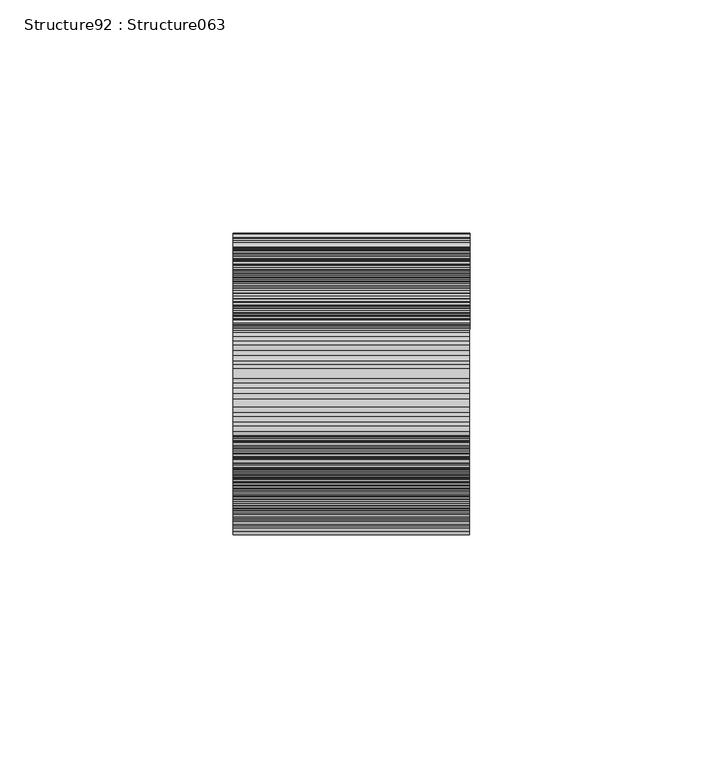
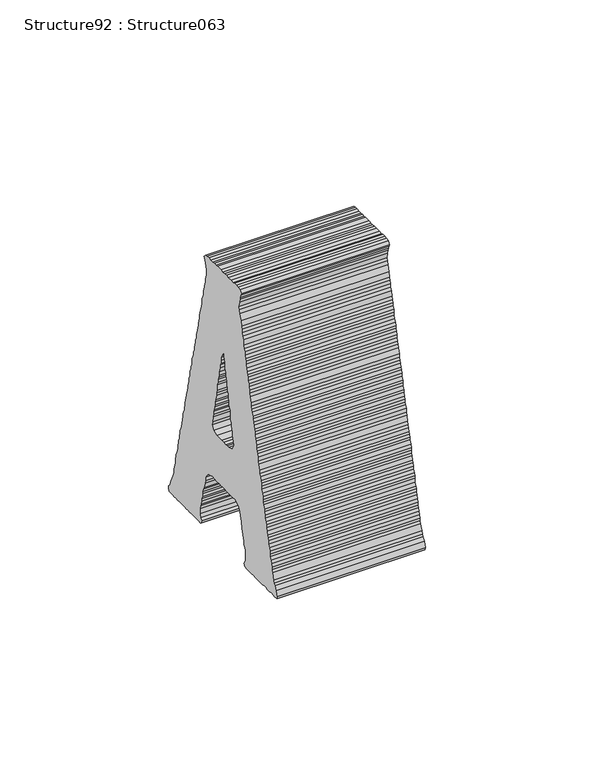
"""IFC4 building model written with IfcOpenShell, lengths in millimetres: proxy geometry, Structure92 : Structure063."""

from ifc_helpers import new_model, si_unit, frame, origin, place, context, project, spatial, polyline, outline, extrude, source, transform, mapped, element, save


def structure92_structure063_1dc17f56(model_context):
    return source(origin(), model_context, "Body", "SweptSolid", [
        extrude(outline(polyline([(0.9094651, 0.0), (2.0811665, -0.5187795), (2.9906316, -0.6522104), (4.1562841, -0.7806598), (5.1991801, -1.1663641), (5.9748585, -1.299795), (7.1504738, -1.690125), (8.1894559, -1.690125), (9.3551083, -2.0804548), (10.2645735, -2.3373539), (11.4362748, -2.5992343), (12.3453841, -2.856489), (13.3818755, -2.9849385), (14.1582655, -3.3752685), (15.4626861, -3.5086994), (16.3721513, -3.5086994), (17.5385154, -3.7705798), (19.491944, -4.4131831), (20.2718921, -4.6750635), (21.3101626, -4.9369439), (22.3470097, -4.9369439), (23.2561191, -5.1988243), (24.4278204, -5.5891542), (25.4700048, -5.9745026), (26.6363689, -5.9745026), (27.4124031, -6.3651884), (28.7175354, -6.6270688), (30.535754, -7.0173988), (31.5743802, -7.1458482), (32.7400327, -7.4077286), (33.6555467, -7.7934329), (35.4741211, -7.7934329), (36.5102567, -7.5361781), (37.5492387, -7.2742977), (38.3288311, -6.8839678), (39.3671015, -6.3651884), (40.4099976, -7.2742977), (40.5395145, -8.1837628), (40.5395145, -9.0978536), (40.2826155, -10.2642177), (40.2826155, -11.3021323), (40.5395145, -12.4731221), (40.4099976, -13.2491562), (40.5395145, -14.1632469), (40.5395145, -16.2390762), (40.2826155, -17.2816164), (40.2826155, -18.319531), (40.5395145, -19.4858951), (40.4099976, -20.6618662), (40.4099976, -22.3470097), (40.2826155, -23.5183552), (40.5395145, -24.422839), (40.5395145, -25.5988102), (40.4099976, -26.5032939), (40.2826155, -27.6696579), (39.2382962, -28.4552992), (38.3288311, -27.9315383), (37.4197218, -27.6696579), (36.6397736, -27.5458341), (35.4741211, -27.2839537), (33.5199809, -26.8936237), (32.6112274, -27.1555041), (31.4448633, -27.4173846), (29.3636968, -28.1934188), (27.545834, -28.4552992), (26.5089869, -28.7121982), (25.3372855, -28.8456291), (24.2943895, -29.1025281), (23.2561191, -29.6216633), (21.3101626, -29.7501128), (20.2718921, -30.0119931), (19.491944, -30.535754), (18.3202426, -30.535754), (17.2816164, -30.9214583), (16.3721513, -31.1783573), (15.3356599, -31.1783573), (14.1582655, -31.4402377), (13.1253323, -31.8305676), (12.2158672, -32.2208975), (11.4362748, -32.3543284), (10.2645735, -32.4827779), (9.3551083, -32.8684823), (8.1894559, -32.8684823), (7.1504738, -33.2588121), (6.2374505, -33.392243), (5.0714422, -33.649142), (3.2475306, -34.2967267), (2.0811665, -34.2967267), (1.1720572, -34.5586071), (0.1334309, -34.8204876), (-1.0382704, -35.3392669), (-1.8178628, -35.4726979), (-2.8568449, -35.7295969), (-3.8990293, -35.8630278), (-5.0653934, -36.2487321), (-5.8471206, -36.5106126), (-7.0166871, -36.5106126), (-8.1826954, -36.9009424), (-8.9644226, -37.0293919), (-10.1364798, -37.4197219), (-11.1690572, -37.5485272), (-12.2115974, -37.6769766), (-12.9915456, -37.938857), (-14.03373, -38.3291869), (-15.3292552, -38.4576365), (-16.3678815, -38.7195168), (-18.1861001, -39.1098467), (-19.3581573, -39.3671016), (-20.2672666, -39.7574315), (-21.4371888, -40.0143304), (-22.2189161, -40.2762109), (-23.1223323, -40.5380913), (-24.1648726, -40.5380913), (-25.465735, -41.052245), (-26.5025822, -41.3141255), (-27.4173846, -41.4475564), (-28.4560108, -41.4475564), (-29.235959, -41.7044554), (-30.5311284, -42.0947853), (-31.3110766, -42.2282162), (-32.3536168, -42.6139205), (-33.5214042, -42.6139205), (-34.4308693, -43.1326999), (-35.3399786, -43.3945803), (-36.37647, -43.3945803), (-37.5424783, -43.6564607), (-38.7202285, -44.0467907), (-39.6236447, -44.3040454), (-40.405372, -44.5609444), (-41.5752942, -44.6943753), (-42.6139205, -45.0847053), (-43.7856218, -45.3465856), (-44.8221132, -45.3465856), (-45.7372714, -45.4750351), (-46.6406876, -45.989189), (-47.812389, -46.2510693), (-48.8510152, -46.5129497), (-49.7601245, -46.5129497), (-50.6731478, -46.9032797), (-52.8777823, -47.5508643), (-53.7929405, -47.9411943), (-54.5689747, -48.3315242), (-55.738897, -49.1125398), (-57.5532016, -49.7597687), (-58.4665807, -49.4978883), (-58.5957419, -48.2030747), (-58.4665807, -47.4270405), (-58.3331498, -46.2510693), (-58.5957419, -45.2131547), (-58.5957419, -44.0467907), (-58.3331498, -43.0042504), (-58.3331498, -42.0947853), (-58.4665807, -41.052245), (-58.4665807, -40.1477613), (-58.5957419, -38.8479663), (-58.5957419, -37.938857), (-58.4665807, -36.9009424), (-58.3331498, -35.7295969), (-58.5957419, -34.8204876), (-58.5957419, -31.8305676), (-58.3331498, -30.6642035), (-57.4297336, -30.1404427), (-56.6480063, -30.535754), (-55.6115149, -30.792653), (-53.3972734, -30.792653), (-52.3586471, -30.792653), (-51.4495378, -30.535754), (-50.6731478, -30.1404427), (-49.3683714, -30.0119931), (-48.4592621, -29.7501128), (-47.5497969, -29.3597829), (-46.6406876, -29.1025281), (-45.6038405, -28.8456291), (-43.2661308, -28.5837487), (-41.5752942, -27.9315383), (-40.2762109, -27.6696579), (-38.9767716, -27.0270546), (-38.1950444, -26.1129639), (-37.4190102, -24.6847194), (-37.6759092, -23.6468048), (-37.6759092, -21.5663499), (-37.5424783, -20.2665549), (-37.5424783, -17.5434968), (-37.6759092, -16.3675257), (-37.4190102, -15.463042), (-37.5424783, -14.4205018), (-37.6759092, -13.3825871), (-37.5424783, -12.4731221), (-37.4190102, -11.1736828), (-37.6759092, -10.3926671), (-38.0676623, -8.8359732), (-38.8476105, -8.0553134), (-40.2762109, -7.0173988), (-41.4422191, -7.0173988), (-42.6139205, -6.7555183), (-44.561656, -6.2367389), (-45.3472973, -5.7176037), (-46.5133056, -5.4557233), (-47.2932538, -5.3272738), (-48.33188, -5.3272738), (-49.3683714, -4.803513), (-50.4126907, -4.6750635), (-51.4495378, -4.546614), (-52.3586471, -4.1609097), (-53.6595096, -3.7705798), (-55.3489229, -3.8990292), (-56.6480063, -4.2893592), (-57.2966585, -4.9369439), (-58.5957419, -4.1609097), (-58.4665807, -2.9849385), (-58.3331498, -1.9470239), (-58.3331498, 0.1334309), (-58.4665807, 1.1663641), (-58.4665807, 2.2092601), (-58.3331498, 3.1183694), (-58.4665807, 4.032816), (-58.4665807, 5.3272738), (-58.3331498, 6.1082894), (-58.4665807, 7.403103), (-58.3331498, 8.1837628), (-58.5957419, 9.2216774), (-58.3331498, 10.3976485), (-58.5957419, 11.5640127), (-58.4665807, 12.4734779), (-58.3331498, 13.5160181), (-58.3331498, 14.5489512), (-57.2966585, 14.9442625), (-56.3875492, 14.6823821), (-55.738897, 14.0301718), (-54.5689747, 13.7732728), (-53.7929405, 13.3825871), (-52.6151903, 12.8638077), (-50.6731478, 11.9543426), (-49.8875066, 11.6924622), (-48.5941162, 11.5640127), (-47.5497969, 11.3021322), (-46.6406876, 11.0452333), (-45.8646534, 10.6549034), (-44.5616561, 10.5264538), (-42.6139205, 10.2642176), (-41.4422191, 9.8738878), (-40.5384471, 9.4835578), (-39.6236447, 9.2216774), (-38.4576364, 9.093228), (-37.4190102, 8.9697599), (-36.5059869, 8.836329), (-35.6004358, 8.3171937), (-34.2956593, 8.1837628), (-33.3922431, 8.0553134), (-32.3536168, 7.9268639), (-31.4405935, 7.5365339), (-30.4019673, 7.146204), (-29.235959, 6.8889492), (-27.5447666, 6.6270688), (-26.3752002, 6.2367389), (-25.203143, 6.1082894), (-24.4235506, 5.846409), (-23.3849244, 5.4607047), (-22.4793732, 5.3272738), (-21.3037579, 4.9369438), (-20.2672666, 4.9369438), (-19.3581573, 4.6750635), (-18.319531, 4.4181645), (-17.1474738, 4.156284), (-15.2018732, 3.6371489), (-14.1632469, 3.3802499), (-13.1207067, 3.3802499), (-12.2115974, 2.9899199), (-11.3024881, 2.5995901), (-10.0012698, 2.5995901), (-9.2270147, 2.0804548), (-8.1826954, 2.0804548), (-7.0166871, 1.9520053), (-5.9745027, 1.4282446), (-5.0653934, 1.4282446), (-4.1619771, 0.9094651), (-2.8568449, 0.7760342), (-1.9473797, 0.7760342), (-0.7817273, 0.2618804), (0.0, 0.0), (0.9094651, 0.0)]), holes=[polyline([(-20.9137838, -13.9013665), (-20.9137838, -16.8912865), (-20.7903157, -18.0576506), (-21.0472147, -19.2286403), (-20.7903157, -20.1381055), (-20.9137838, -21.0475706), (-20.2672666, -22.9945945), (-18.5817672, -23.6468048), (-17.2809048, -23.3849243), (-16.3678815, -23.1280254), (-15.4623303, -22.866145), (-14.1632469, -22.9945945), (-13.2480888, -22.4804406), (-12.2115974, -22.3470097), (-11.3024881, -22.2185603), (-10.393023, -21.8282304), (-9.3508386, -21.6947994), (-8.3122123, -21.6947994), (-7.146204, -21.5663499), (-6.3644768, -21.1760201), (-5.3276296, -20.9187653), (-4.2854452, -20.9187653), (-3.117302, -20.3999858), (-1.9473797, -20.3999858), (-1.0382704, -20.009656), (-0.2561874, -19.8762251), (1.0389821, -19.7477755), (2.0811665, -19.4858951), (3.1180136, -19.2286403), (4.0274787, -19.1001908), (5.0714422, -19.1001908), (6.1082894, -18.5814114), (7.0177545, -18.4479805), (8.1894559, -18.4479805), (9.2216774, -18.0576506), (10.1368356, -17.7957702), (11.0463007, -17.7957702), (10.1368356, -17.1531669), (9.0928721, -16.7578556), (8.056025, -16.6294061), (6.8900167, -16.6294061), (6.1082894, -16.1106266), (4.9365881, -15.9771957), (3.1180136, -15.463042), (1.8189302, -15.3296111), (0.9094651, -15.2011615), (0.0, -14.9392811), (-1.0382704, -14.8108316), (-2.2078369, -14.4205018), (-4.2854452, -14.2870708), (-5.3276296, -14.0347974), (-6.3644768, -13.9013665), (-8.1826954, -13.5110367), (-9.2270147, -12.9922572), (-10.2638619, -12.9922572), (-11.1690572, -12.7303768), (-12.3446725, -12.6015715), (-13.1207067, -12.216223), (-14.286715, -12.216223), (-15.4623303, -11.8209117), (-17.2809048, -11.5640127), (-18.5817672, -11.3021323), (-20.1377496, -12.0827921), (-20.9137838, -13.9013665)])]), frame((-56111.5720734, 291157.0961008, -317.0048136), z_axis=(-0.9999998917542984, 0.00046528635450596156, 0.0), x_axis=(0.0, 0.0, 1.0)), (0.0, 0.0, 1.0), 50.8),
    ])


if __name__ == "__main__":
    model = new_model("IFC4")
    model_context = context("Model", 3, world=origin())
    ifc_project = project(units=[si_unit("LENGTHUNIT", "METRE", prefix="MILLI")], contexts=[model_context])
    site = spatial("IfcSite", under=ifc_project)
    building = spatial("IfcBuilding", under=site)
    placement = place(None, origin())
    structure92_structure063_shape = structure92_structure063_1dc17f56(model_context)
    element("IfcBuildingElementProxy", 1, Name="Structure92 : Structure063", ObjectType="Structure92 : Structure063", at=placement, inside=building, context=model_context, shape_type="MappedRepresentation", body=[
        mapped(structure92_structure063_shape, transform((0.0, 0.0, 0.0), x_axis=(1.0, 0.0, 0.0), y_axis=(0.0, 1.0, 0.0), z_axis=(0.0, 0.0, 1.0))),
    ])
    save(model, "model.ifc")

# Revit data of these elements
# Type "Structure92 : Structure063"
#   NameOverride = "Structure063"
# Element 1 (IfcBuildingElementProxy, "Structure92 : Structure063")
#   Materials on its faces: "BRUSHED ALUMINUM LETTERING"
# Materials
#   "BRUSHED ALUMINUM LETTERING": class "Unassigned", colour RGB 169 181 186, transparency 0, Cost = 0
